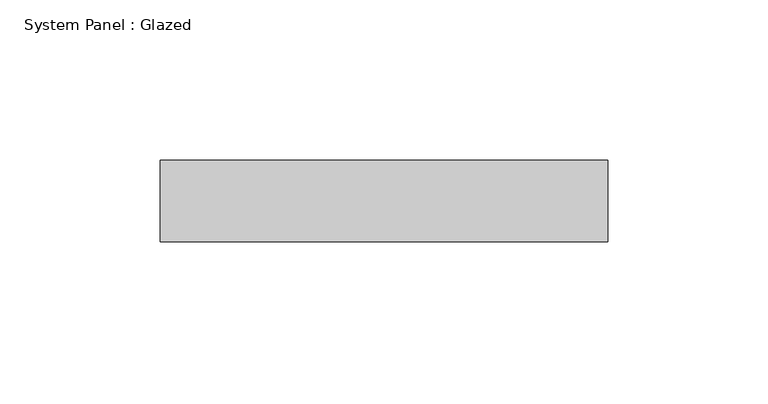
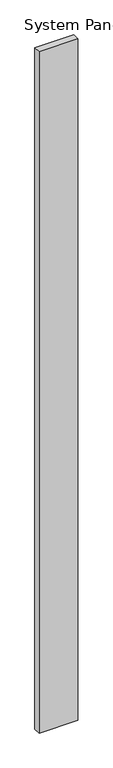
"""IFC4 building model written with IfcOpenShell, lengths in millimetres: plate geometry, System Panel : Glazed."""

from ifc_helpers import new_model, si_unit, origin, origin_with_axes, place, context, project, spatial, polyline, outline, extrude, source, transform, mapped, element, save


def system_panel_glazed_a3432af0(model_context):
    return source(origin(), model_context, "Body", "SweptSolid", [
        extrude(outline(polyline([(69.649919, 19.05), (-69.649919, 19.05), (-69.649919, 44.45), (69.649919, 44.45), (69.649919, 19.05)])), origin_with_axes(), (0.0, 0.0, 1.0), 2578.1),
    ])


if __name__ == "__main__":
    model = new_model("IFC4")
    model_context = context("Model", 3, world=origin())
    ifc_project = project(units=[si_unit("LENGTHUNIT", "METRE", prefix="MILLI")], contexts=[model_context])
    site = spatial("IfcSite", under=ifc_project)
    building = spatial("IfcBuilding", under=site)
    placement = place(None, origin())
    system_panel_glazed_shape = system_panel_glazed_a3432af0(model_context)
    element("IfcPlate", 1, ObjectType="System Panel : Glazed", at=placement, inside=building, context=model_context, shape_type="MappedRepresentation", body=[
        mapped(system_panel_glazed_shape, transform((0.0, 0.0, 0.0), x_axis=(1.0, 0.0, 0.0), y_axis=(0.0, 1.0, 0.0), z_axis=(0.0, 0.0, 1.0))),
    ])
    save(model, "model.ifc")

# Revit data of these elements
# Type "System Panel : Glazed"
#   Construction Type Id = "GSP4R"
#   Analytic Construction = "1/8 in Pilkington single glazing"
#   Visual Light Transmittance = 0.9
#   Solar Heat Gain Coefficient = 0.86
#   Heat Transfer Coefficient (U) = 1.18115 BTU/(h·ft²·°F)
#   Define Thermal Properties by = 1
# Element 1 (IfcPlate, "System Panel : Glazed")
#   Materials on its faces: "Glass"
# Materials
#   "Glass": class "Glass", colour RGB 0 128 192, transparency 0.75, Description = "Soda Lime Glass", Cost = 0
